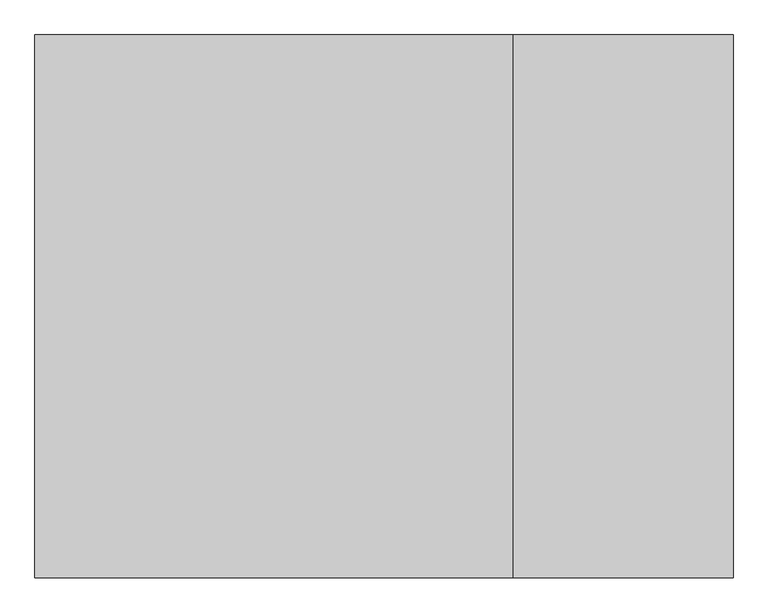
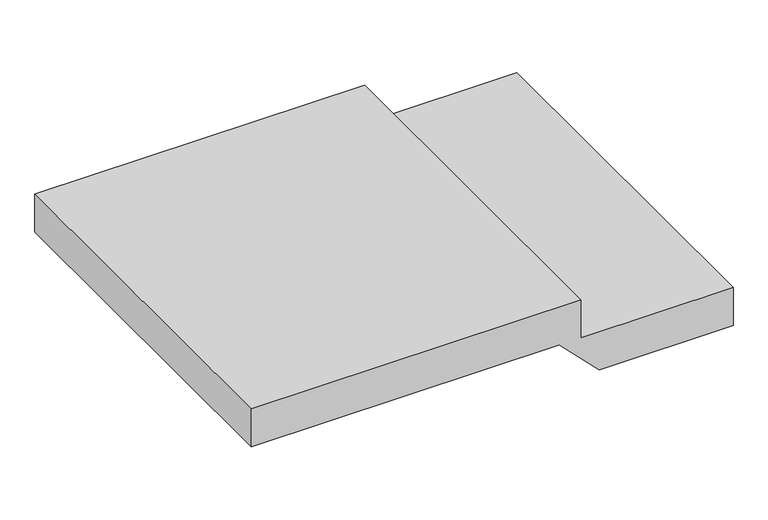
"""IFC4 building model written with IfcOpenShell, lengths in millimetres: proxy geometry, 벽 5 : 벽 1."""

from ifc_helpers import new_model, si_unit, frame, origin, place, context, project, spatial, polyline, outline, extrude, source, transform, mapped, element, save


def generic_models_a06d278e(model_context):
    return source(origin(), model_context, "Body", "SweptSolid", [
        extrude(outline(polyline([(599.905241, 43602.1335861), (599.905241, 42370.0), (449.905241, 42370.0), (449.905241, 43520.0), (299.905241, 43670.0), (299.905241, 44170.4893475), (449.905241, 44170.4893475), (449.905241, 43602.1335861), (599.905241, 43602.1335861)])), frame((0.0, 21999.5208589, 0.0), z_axis=(0.0, 1.0, 0.0), x_axis=(0.0, 0.0, 1.0)), (0.0, 0.0, 1.0), 1400.0),
    ])


if __name__ == "__main__":
    model = new_model("IFC4")
    model_context = context("Model", 3, world=origin())
    ifc_project = project(units=[si_unit("LENGTHUNIT", "METRE", prefix="MILLI")], contexts=[model_context])
    site = spatial("IfcSite", under=ifc_project)
    building = spatial("IfcBuilding", under=site)
    placement = place(None, origin())
    generic_models_shape = generic_models_a06d278e(model_context)
    element("IfcBuildingElementProxy", 1, Name="벽 5 : 벽 1", ObjectType="벽 5 : 벽 1", at=placement, inside=building, context=model_context, shape_type="MappedRepresentation", body=[
        mapped(generic_models_shape, transform((0.0, 0.0, 0.0), x_axis=(1.0, 0.0, 0.0), y_axis=(0.0, 1.0, 0.0), z_axis=(0.0, 0.0, 1.0))),
    ])
    save(model, "model.ifc")

# Revit data of these elements
# Element 1 (IfcBuildingElementProxy, "벽 5 : 벽 1")
#   Materials on its faces: "A03AC032-00007_Structural Concrete_Type1_25MPa-30Mpa"
# Materials
#   "A03AC032-00007_Structural Concrete_Type1_25MPa-30Mpa": class "Concrete", colour RGB 176 176 176, transparency 0, Keynote = "09910.A1", Description = "Reinf. Conc.", W00) Work Master Code = "A03AC032-00007", W01) Work Master_Lv1 = "Concrete Work", W02) Work Master_Lv2 = "Substructure Work", W03) Work Master_Spec.1 = "Structural Concrete", W04) Work Master_Spec.2 = "Cement Type-1", W05) Work Master_Spec.3 = "25MPa < F'c (Cylinder Strength) ≤ 30MPa", Cost = 0
